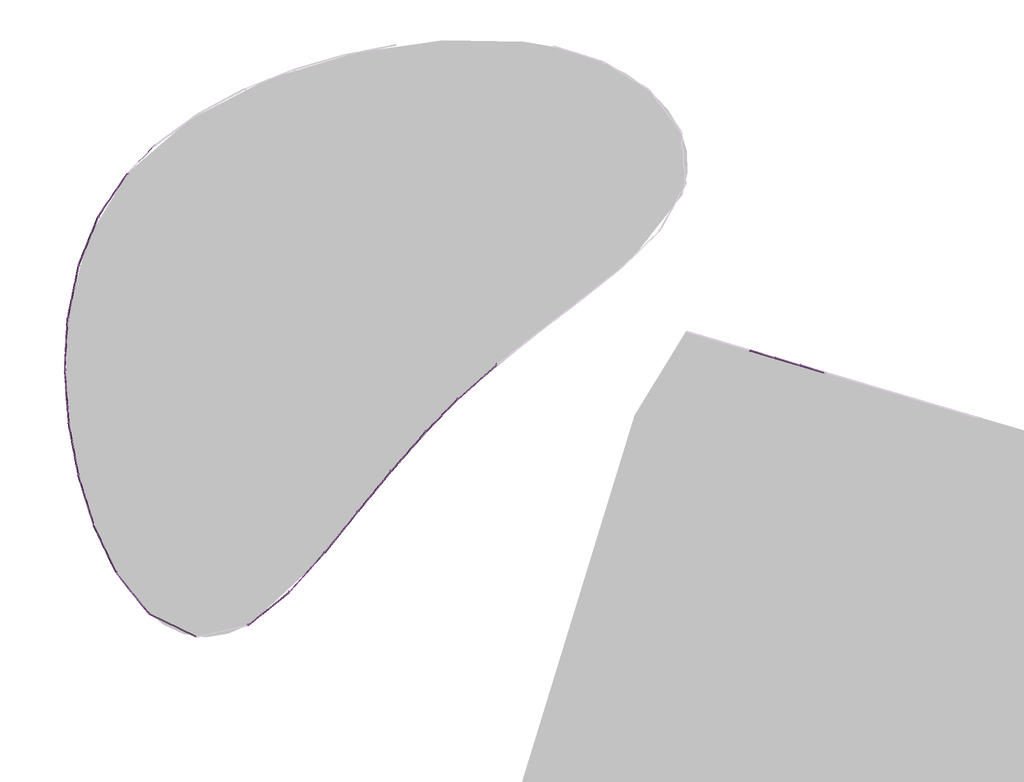
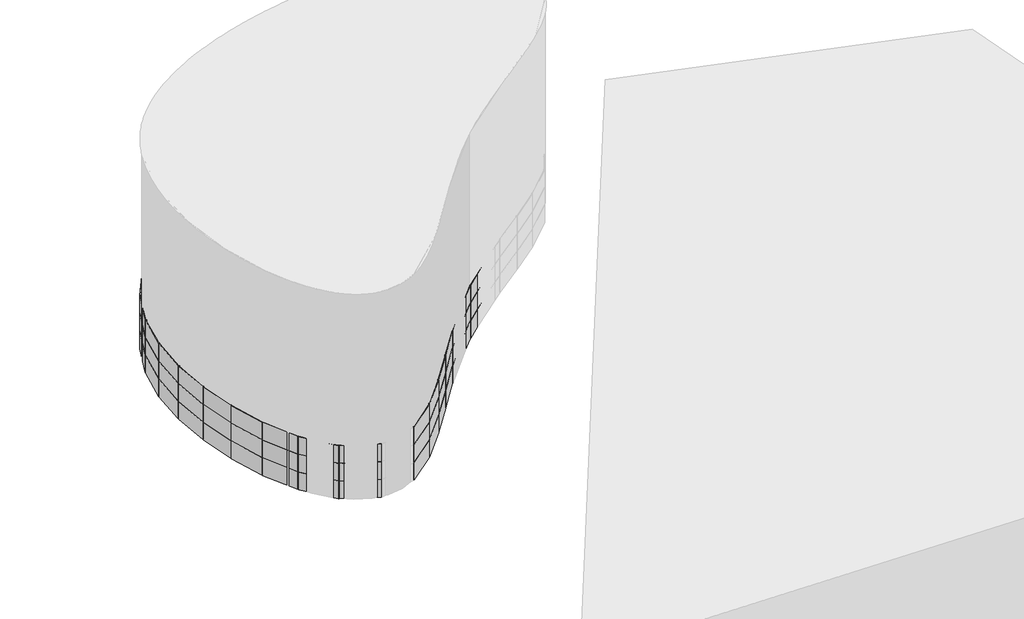
# One storey, part 3 of 5: 58 plates, 54 members.
"""IFC4 building model written with IfcOpenShell, lengths in millimetres."""

import ifcopenshell
import ifcopenshell.guid

model = None  # the IFC model being written
_history = None  # IfcOwnerHistory: only IFC2X3 demands one
_inside = {}  # id of a spatial element -> (the spatial element, [elements in it])
_under = {}  # id of a project, library or spatial element -> (it, [spatial elements below it])
_declared = {}  # id of a project -> (the project, [libraries it declares])
_typed = {}  # id of a type object -> (the type object, [elements of that type])
_made_of = {}  # id of a material, layer set ... -> (it, [elements and type objects made of it])


def new_model(schema):
    """Start an empty IFC model of exactly this schema.

    Asked for "IFC4X3", IfcOpenShell would pick the latest addendum, in which some entities
    have other attributes; the version numbers below select the first issue.
    IFC2X3 requires an IfcOwnerHistory on every rooted entity: one is made here for all.
    """
    global model, _history
    if schema == "IFC4X3":
        model = ifcopenshell.file(schema_version=(4, 3, 0, 0))
    else:
        model = ifcopenshell.file(schema=schema)
    _inside.clear()
    _under.clear()
    _declared.clear()
    _typed.clear()
    _made_of.clear()
    _history = None
    if model.schema == "IFC2X3":
        org = make("IfcOrganization", Name="unknown")
        user = make(
            "IfcPersonAndOrganization",
            ThePerson=make("IfcPerson", FamilyName="unknown"),
            TheOrganization=org,
        )
        app = make(
            "IfcApplication",
            ApplicationDeveloper=org,
            Version="unknown",
            ApplicationFullName="unknown",
            ApplicationIdentifier="unknown",
        )
        _history = make(
            "IfcOwnerHistory",
            OwningUser=user,
            OwningApplication=app,
            ChangeAction="ADDED",
            CreationDate=0,
        )
    return model


def make(cls, **values):
    """One entity of the class cls with the attributes given. An attribute that is None is left unset."""
    return model.create_entity(
        cls, **{name: value for name, value in values.items() if value is not None}
    )


def rooted(cls, **values):
    """An entity with a GlobalId (a new one), such as an element, a storey or a relation."""
    return make(cls, GlobalId=ifcopenshell.guid.new(), OwnerHistory=_history, **values)


def si_unit(unit_type, name, prefix=None):
    """IfcSIUnit, for example si_unit("LENGTHUNIT", "METRE", prefix="MILLI")."""
    return make("IfcSIUnit", UnitType=unit_type, Prefix=prefix, Name=name)


def assignment(units):
    """IfcUnitAssignment: the units of a project."""
    return None if units is None else make("IfcUnitAssignment", Units=units)


def point(xyz):
    """IfcCartesianPoint."""
    return None if xyz is None else make("IfcCartesianPoint", Coordinates=xyz)


def direction(xyz):
    """IfcDirection."""
    return None if xyz is None else make("IfcDirection", DirectionRatios=xyz)


def frame(location, z_axis=None, x_axis=None):
    """IfcAxis2Placement3D, a coordinate frame: its origin and axes. An axis left out is left unset."""
    return make(
        "IfcAxis2Placement3D",
        Location=point(location),
        Axis=direction(z_axis),
        RefDirection=direction(x_axis),
    )


def frame_2d(location, x_axis=None):
    """IfcAxis2Placement2D, a coordinate frame in the plane: its origin and x axis."""
    return make(
        "IfcAxis2Placement2D", Location=point(location), RefDirection=direction(x_axis)
    )


def origin():
    """The frame at (0, 0, 0) with its axes left unset."""
    return frame((0.0, 0.0, 0.0))


def origin_with_axes():
    """The frame at (0, 0, 0) with the z axis (0, 0, 1) and the x axis (1, 0, 0) written out."""
    return frame((0.0, 0.0, 0.0), z_axis=(0.0, 0.0, 1.0), x_axis=(1.0, 0.0, 0.0))


def origin_2d():
    """The frame at (0, 0) in the plane with its x axis left unset."""
    return frame_2d((0.0, 0.0))


def place(relative_to, where):
    """IfcLocalPlacement: puts the frame where relative to a parent placement (None: the world)."""
    return make(
        "IfcLocalPlacement", PlacementRelTo=relative_to, RelativePlacement=where
    )


def context(
    kind, dimensions, precision=None, world=None, true_north=None, identifier=None
):
    """IfcGeometricRepresentationContext, for example the 3D "Model" context."""
    return make(
        "IfcGeometricRepresentationContext",
        ContextIdentifier=identifier,
        ContextType=kind,
        CoordinateSpaceDimension=dimensions,
        Precision=precision,
        WorldCoordinateSystem=world,
        TrueNorth=true_north,
    )


def project(units=None, contexts=None):
    """IfcProject with its units and contexts."""
    return rooted(
        "IfcProject",
        Name="project",
        RepresentationContexts=contexts,
        UnitsInContext=assignment(units),
    )


def spatial(cls, under=None, at=None, **own):
    """A site, building, storey or space (cls), placed at a placement, below another one or the project."""
    s = rooted(cls, ObjectPlacement=at, **own)
    if under is not None:
        _under.setdefault(under.id(), (under, []))[1].append(s)
    return s


def polyline(points):
    """IfcPolyline through the points."""
    return make("IfcPolyline", Points=[point(p) for p in points])


def circle_curve(where, radius):
    """IfcCircle in the frame where."""
    return make("IfcCircle", Position=where, Radius=radius)


def trimmed(basis, trim1, trim2, sense, master):
    """IfcTrimmedCurve: the piece of a basis curve between two trims."""
    return make(
        "IfcTrimmedCurve",
        BasisCurve=basis,
        Trim1=trim1,
        Trim2=trim2,
        SenseAgreement=sense,
        MasterRepresentation=master,
    )


def segment(curve, same_sense, transition):
    """IfcCompositeCurveSegment."""
    return make(
        "IfcCompositeCurveSegment",
        Transition=transition,
        SameSense=same_sense,
        ParentCurve=curve,
    )


def composite_curve(segments, self_intersect=None):
    """IfcCompositeCurve: segments joined end to end."""
    return make("IfcCompositeCurve", Segments=segments, SelfIntersect=self_intersect)


def outline(outer, holes=None, kind="AREA"):
    """IfcArbitraryClosedProfileDef: a profile drawn as a closed curve; with holes, ...WithVoids."""
    if holes is None:
        return make("IfcArbitraryClosedProfileDef", ProfileType=kind, OuterCurve=outer)
    return make(
        "IfcArbitraryProfileDefWithVoids",
        ProfileType=kind,
        OuterCurve=outer,
        InnerCurves=holes,
    )


def extrude(swept, where, along, depth):
    """IfcExtrudedAreaSolid: the profile swept, set in the frame where, extruded along a direction by depth."""
    return make(
        "IfcExtrudedAreaSolid",
        SweptArea=swept,
        Position=where,
        ExtrudedDirection=direction(along),
        Depth=depth,
    )


def shape(context_of_items, identifier, shape_type, items):
    """IfcShapeRepresentation: the items that make up one representation, for example the "Body"."""
    return make(
        "IfcShapeRepresentation",
        ContextOfItems=context_of_items,
        RepresentationIdentifier=identifier,
        RepresentationType=shape_type,
        Items=items,
    )


def source(mapping_origin, context_of_items, identifier, shape_type, items):
    """IfcRepresentationMap: a shape defined once, which mapped items show again and again."""
    return make(
        "IfcRepresentationMap",
        MappingOrigin=mapping_origin,
        MappedRepresentation=shape(context_of_items, identifier, shape_type, items),
    )


def transform(
    local_origin,
    x_axis=None,
    y_axis=None,
    z_axis=None,
    scale=None,
    scale2=None,
    scale3=None,
    uniform=True,
):
    """IfcCartesianTransformationOperator3D, or its non-uniform kind. x_axis, y_axis, z_axis: its Axis1, 2, 3."""
    if uniform:
        return make(
            "IfcCartesianTransformationOperator3D",
            Axis1=direction(x_axis),
            Axis2=direction(y_axis),
            LocalOrigin=point(local_origin),
            Scale=scale,
            Axis3=direction(z_axis),
        )
    return make(
        "IfcCartesianTransformationOperator3DnonUniform",
        Axis1=direction(x_axis),
        Axis2=direction(y_axis),
        LocalOrigin=point(local_origin),
        Scale=scale,
        Axis3=direction(z_axis),
        Scale2=scale2,
        Scale3=scale3,
    )


def mapped(mapping_source, mapping_target):
    """IfcMappedItem: shows the shape of a source again, moved by a transform."""
    return make(
        "IfcMappedItem", MappingSource=mapping_source, MappingTarget=mapping_target
    )


def made_of(thing, what):
    """Note that an element or type object is made of a material, layer set ...; save() writes the relation."""
    if what is not None:
        _made_of.setdefault(what.id(), (what, []))[1].append(thing)
    return thing


def element(
    cls,
    number,
    at=None,
    inside=None,
    cuts=None,
    type_object=None,
    material=None,
    context=None,
    identifier="Body",
    shape_type=None,
    held_by="IfcProductDefinitionShape",
    body=None,
    shapes=None,
    **own,
):
    """One element of the class cls, such as IfcWall. Its Tag is "e" and its number.

    at: its placement. inside: the storey or other place that contains it. cuts: it is an
    opening in that element (IfcRelVoidsElement). A single representation is given by context,
    identifier, shape_type and body (its items); several are given by shapes. held_by: the class
    of the entity that holds the representations. save() writes the other relations.
    """
    e = rooted(cls, Tag="e%d" % number, ObjectPlacement=at, **own)
    if body is not None:
        shapes = [shape(context, identifier, shape_type, body)]
    if shapes is not None:
        e.Representation = make(held_by, Representations=shapes)
    if inside is not None:
        _inside.setdefault(inside.id(), (inside, []))[1].append(e)
    if cuts is not None:
        rooted(
            "IfcRelVoidsElement", RelatingBuildingElement=cuts, RelatedOpeningElement=e
        )
    if type_object is not None:
        _typed.setdefault(type_object.id(), (type_object, []))[1].append(e)
    return made_of(e, material)


def aggregate(whole, parts):
    """IfcRelAggregates: a whole, such as a stair, and the parts it consists of."""
    return rooted("IfcRelAggregates", RelatingObject=whole, RelatedObjects=parts)


def save(model, path):
    """Write the relations noted so far, then the file.

    IfcRelAggregates (storeys below a building ...), IfcRelContainedInSpatialStructure (elements
    in a storey), IfcRelDefinesByType, IfcRelAssociatesMaterial and IfcRelDeclares: one each for
    every whole, place, type object, material and project.
    """
    for whole, parts in _under.values():
        aggregate(whole, parts)
    for where, things in _inside.values():
        rooted(
            "IfcRelContainedInSpatialStructure",
            RelatedElements=things,
            RelatingStructure=where,
        )
    for kind, things in _typed.values():
        rooted("IfcRelDefinesByType", RelatedObjects=things, RelatingType=kind)
    for what, things in _made_of.values():
        rooted("IfcRelAssociatesMaterial", RelatedObjects=things, RelatingMaterial=what)
    for by, libraries in _declared.values():
        rooted("IfcRelDeclares", RelatingContext=by, RelatedDefinitions=libraries)
    model.write(path)


def montante_circular_25_mm_raio_36e581cf(model_context):
    return source(origin(), model_context, "Body", "SweptSolid", [
        extrude(outline(composite_curve([segment(trimmed(circle_curve(origin_2d(), 25.0), [point((25.0, 0.0))], [point((-25.0, 0.0))], False, "CARTESIAN"), True, "CONTINUOUS"), segment(trimmed(circle_curve(origin_2d(), 25.0), [point((-25.0, 0.0))], [point((25.0, 0.0))], False, "CARTESIAN"), True, "CONTINUOUS")], self_intersect=False)), frame((0.0, 0.0, -1500.0), z_axis=(0.0, 0.0, 1.0), x_axis=(1.0, 0.0, 0.0)), (0.0, 0.0, 1.0), 1500.0),
    ])


def montante_circular_25_mm_raio_ce826986(model_context):
    return source(origin(), model_context, "Body", "SweptSolid", [
        extrude(outline(composite_curve([segment(trimmed(circle_curve(frame_2d((-25.0, 0.0)), 25.0), [point((0.0, 0.0))], [point((-50.0, 0.0))], False, "CARTESIAN"), True, "CONTINUOUS"), segment(trimmed(circle_curve(frame_2d((-25.0, 0.0)), 25.0), [point((-50.0, 0.0))], [point((0.0, 0.0))], False, "CARTESIAN"), True, "CONTINUOUS")], self_intersect=False)), frame((0.0, 0.0, -1500.0), z_axis=(0.0, 0.0, 1.0), x_axis=(1.0, 0.0, 0.0)), (0.0, 0.0, 1.0), 1500.0),
    ])


def painel_do_sistema_ee4f1c4d(model_context):
    return source(origin(), model_context, "Body", "SweptSolid", [
        extrude(outline(polyline([(1487.5000075, 24.5), (-1487.5000075, 24.5), (-1487.5000075, 49.5), (1487.5000075, 49.5), (1487.5000075, 24.5)])), origin_with_axes(), (0.0, 0.0, 1.0), 1500.0),
    ])


def painel_do_sistema_5ef9eced(model_context):
    return source(origin(), model_context, "Body", "SweptSolid", [
        extrude(outline(polyline([(1475.0, 24.5), (-1475.0, 24.5), (-1475.0, 49.5), (1475.0, 49.5), (1475.0, 24.5)])), origin_with_axes(), (0.0, 0.0, 1.0), 1500.0),
    ])


def painel_do_sistema_619734db(model_context):
    return source(origin(), model_context, "Body", "SweptSolid", [
        extrude(outline(polyline([(1462.5000305, -49.5), (-1462.5000305, -49.5), (-1462.5000305, -24.5), (1462.5000305, -24.5), (1462.5000305, -49.5)])), origin_with_axes(), (0.0, 0.0, 1.0), 1500.0),
    ])


def painel_do_sistema_9c2734b9(model_context):
    return source(origin(), model_context, "Body", "SweptSolid", [
        extrude(outline(polyline([(1462.5000336, -49.5), (-1462.5000336, -49.5), (-1462.5000336, -24.5), (1462.5000336, -24.5), (1462.5000336, -49.5)])), origin_with_axes(), (0.0, 0.0, 1.0), 1500.0),
    ])


def painel_do_sistema_85ccde5d(model_context):
    return source(origin(), model_context, "Body", "SweptSolid", [
        extrude(outline(polyline([(1475.0, -49.5), (-1475.0, -49.5), (-1475.0, -24.5), (1475.0, -24.5), (1475.0, -49.5)])), origin_with_axes(), (0.0, 0.0, 1.0), 1500.0),
    ])


def painel_do_sistema_91df381f(model_context):
    return source(origin(), model_context, "Body", "SweptSolid", [
        extrude(outline(polyline([(1110.3819696, -49.5), (-1110.3819696, -49.5), (-1110.3819696, -24.5), (1110.3819696, -24.5), (1110.3819696, -49.5)])), origin_with_axes(), (0.0, 0.0, 1.0), 1500.0),
    ])


def painel_do_sistema_bfc8fefc(model_context):
    return source(origin(), model_context, "Body", "SweptSolid", [
        extrude(outline(polyline([(1275.8375317, -49.5), (-1275.8375317, -49.5), (-1275.8375317, -24.5), (1275.8375317, -24.5), (1275.8375317, -49.5)])), origin_with_axes(), (0.0, 0.0, 1.0), 1500.0),
    ])


model = new_model("IFC4")

# Units and contexts
model_context = context("Model", 3, world=origin())
ifc_project = project(units=[si_unit("LENGTHUNIT", "METRE", prefix="MILLI")], contexts=[model_context])

# Site, building, storey
site = spatial("IfcSite", under=ifc_project)
building = spatial("IfcBuilding", under=site)
storey = spatial("IfcBuildingStorey", under=building, Name="Nível 1", Elevation=0.0)

# Members
placement = place(None, origin())
montante_circular_25_mm_raio_shape = montante_circular_25_mm_raio_36e581cf(model_context)
element("IfcMember", 1, ObjectType="Montante circular : 25 mm Raio", at=placement, inside=storey, context=model_context, shape_type="MappedRepresentation", body=[
    mapped(montante_circular_25_mm_raio_shape, transform((-73.9726554, 31091.8210426, 3000.000015), x_axis=(0.0, 0.0, 1.0), y_axis=(0.28318378939534855, 0.9590656606425293, 0.0), z_axis=(-0.9590656606425293, 0.28318378939534855, 0.0))),
])
element("IfcMember", 2, ObjectType="Montante circular : 25 mm Raio", at=placement, inside=storey, context=model_context, shape_type="MappedRepresentation", body=[
    mapped(montante_circular_25_mm_raio_shape, transform((-1512.5711463, 31516.5967267, 3000.000015), x_axis=(0.0, 0.0, 1.0), y_axis=(0.28318378939534655, 0.9590656606425297, 0.0), z_axis=(-0.9590656606425296, 0.2831837893953465, 0.0))),
])
element("IfcMember", 3, ObjectType="Montante circular : 25 mm Raio", at=placement, inside=storey, context=model_context, shape_type="MappedRepresentation", body=[
    mapped(montante_circular_25_mm_raio_shape, transform((-2951.1696373, 31941.3724108, 3000.000015), x_axis=(0.0, 0.0, 1.0), y_axis=(0.2831837893953519, 0.9590656606425282, 0.0), z_axis=(-0.9590656606425281, 0.2831837893953518, 0.0))),
])
element("IfcMember", 4, ObjectType="Montante circular : 25 mm Raio", at=placement, inside=storey, context=model_context, shape_type="MappedRepresentation", body=[
    mapped(montante_circular_25_mm_raio_shape, transform((-40020.7762885, 39520.8946952, 1500.0), x_axis=(-0.46558849269393926, -0.8850013307735677, 0.0), y_axis=(-0.8850013307735677, 0.46558849269393926, 0.0), z_axis=(0.0, 0.0, -1.0))),
])
element("IfcMember", 5, ObjectType="Montante circular : 25 mm Raio", at=placement, inside=storey, context=model_context, shape_type="MappedRepresentation", body=[
    mapped(montante_circular_25_mm_raio_shape, transform((-41145.2595981, 36739.6113068, 1500.0), x_axis=(-0.2854090553713671, -0.9584057966811469, 0.0), y_axis=(-0.9584057966811469, 0.2854090553713671, 0.0), z_axis=(0.0, 0.0, -1.0))),
])
element("IfcMember", 6, ObjectType="Montante circular : 25 mm Raio", at=placement, inside=storey, context=model_context, shape_type="MappedRepresentation", body=[
    mapped(montante_circular_25_mm_raio_shape, transform((-41757.3897475, 33802.725766, 1500.0), x_axis=(-0.12631233821712984, -0.9919905207279561, 0.0), y_axis=(-0.9919905207279561, 0.12631233821712984, 0.0), z_axis=(0.0, 0.0, -1.0))),
])
element("IfcMember", 7, ObjectType="Montante circular : 25 mm Raio", at=placement, inside=storey, context=model_context, shape_type="MappedRepresentation", body=[
    mapped(montante_circular_25_mm_raio_shape, transform((-41927.7364355, 30807.566003, 1500.0), x_axis=(0.00926833746122375, -0.999957048037917, 0.0), y_axis=(-0.999957048037917, -0.00926833746122375, 0.0), z_axis=(0.0, 0.0, -1.0))),
])
element("IfcMember", 8, ObjectType="Montante circular : 25 mm Raio", at=placement, inside=storey, context=model_context, shape_type="MappedRepresentation", body=[
    mapped(montante_circular_25_mm_raio_shape, transform((-41719.5366875, 27814.7992454, 1500.0), x_axis=(0.12720739477424994, -0.9918761408133316, 0.0), y_axis=(-0.9918761408133316, -0.12720739477424994, 0.0), z_axis=(0.0, 0.0, -1.0))),
])
element("IfcMember", 9, ObjectType="Montante circular : 25 mm Raio", at=placement, inside=storey, context=model_context, shape_type="MappedRepresentation", body=[
    mapped(montante_circular_25_mm_raio_shape, transform((-41172.4912602, 24865.0973452, 1500.0), x_axis=(0.2368789337610514, -0.9715391761222125, 0.0), y_axis=(-0.9715391761222125, -0.2368789337610514, 0.0), z_axis=(0.0, 0.0, -1.0))),
])
element("IfcMember", 10, ObjectType="Montante circular : 25 mm Raio", at=placement, inside=storey, context=model_context, shape_type="MappedRepresentation", body=[
    mapped(montante_circular_25_mm_raio_shape, transform((-39014.8508906, 19282.6093761, 1500.0), x_axis=(0.5079873162147127, -0.8613645491689181, 0.0), y_axis=(-0.8613645491689181, -0.5079873162147127, 0.0), z_axis=(0.0, 0.0, -1.0))),
])
element("IfcMember", 11, ObjectType="Montante circular : 25 mm Raio", at=placement, inside=storey, context=model_context, shape_type="MappedRepresentation", body=[
    mapped(montante_circular_25_mm_raio_shape, transform((-37150.2365801, 16932.4575783, 1500.0), x_axis=(0.7466685294931724, -0.665196292130754, 0.0), y_axis=(-0.665196292130754, -0.7466685294931724, 0.0), z_axis=(0.0, 0.0, -1.0))),
])
element("IfcMember", 12, ObjectType="Montante circular : 25 mm Raio", at=placement, inside=storey, context=model_context, shape_type="MappedRepresentation", body=[
    mapped(montante_circular_25_mm_raio_shape, transform((-31525.1733328, 16282.9834173, 1500.0), x_axis=(0.8701634838175947, 0.492763139277307, 0.0), y_axis=(0.492763139277307, -0.8701634838175947, 0.0), z_axis=(0.0, 0.0, -1.0))),
])
element("IfcMember", 13, ObjectType="Montante circular : 25 mm Raio", at=placement, inside=storey, context=model_context, shape_type="MappedRepresentation", body=[
    mapped(montante_circular_25_mm_raio_shape, transform((-29189.3459235, 18165.5110569, 1500.0), x_axis=(0.7046961293095542, 0.7095092426009207, 0.0), y_axis=(0.7095092426009207, -0.7046961293095542, 0.0), z_axis=(0.0, 0.0, -1.0))),
])
element("IfcMember", 14, ObjectType="Montante circular : 25 mm Raio", at=placement, inside=storey, context=model_context, shape_type="MappedRepresentation", body=[
    mapped(montante_circular_25_mm_raio_shape, transform((-27187.2576877, 20399.7095029, 1500.0), x_axis=(0.6410206876840714, 0.7675236009146822, 0.0), y_axis=(0.7675236009146822, -0.6410206876840714, 0.0), z_axis=(0.0, 0.0, -1.0))),
])
element("IfcMember", 15, ObjectType="Montante circular : 25 mm Raio", at=placement, inside=storey, context=model_context, shape_type="MappedRepresentation", body=[
    mapped(montante_circular_25_mm_raio_shape, transform((-25293.7553869, 22726.6493467, 1500.0), x_axis=(0.6272671926241681, 0.7788041275297628, 0.0), y_axis=(0.7788041275297628, -0.6272671926241681, 0.0), z_axis=(0.0, 0.0, -1.0))),
])
element("IfcMember", 16, ObjectType="Montante circular : 25 mm Raio", at=placement, inside=storey, context=model_context, shape_type="MappedRepresentation", body=[
    mapped(montante_circular_25_mm_raio_shape, transform((-23394.8086307, 25049.1482632, 1500.0), x_axis=(0.6426798456549805, 0.7661348549628131, 0.0), y_axis=(0.7661348549628131, -0.6426798456549805, 0.0), z_axis=(0.0, 0.0, -1.0))),
])
element("IfcMember", 17, ObjectType="Montante circular : 25 mm Raio", at=placement, inside=storey, context=model_context, shape_type="MappedRepresentation", body=[
    mapped(montante_circular_25_mm_raio_shape, transform((-21416.0981725, 27304.0772915, 1500.0), x_axis=(0.6795654424505699, 0.7336148917701719, 0.0), y_axis=(0.7336148917701719, -0.6795654424505699, 0.0), z_axis=(0.0, 0.0, -1.0))),
])
element("IfcMember", 18, ObjectType="Montante circular : 25 mm Raio", at=placement, inside=storey, context=model_context, shape_type="MappedRepresentation", body=[
    mapped(montante_circular_25_mm_raio_shape, transform((-40020.7762885, 39520.8946952, 3000.0), x_axis=(-0.46558849269393926, -0.8850013307735677, 0.0), y_axis=(-0.8850013307735677, 0.46558849269393926, 0.0), z_axis=(0.0, 0.0, -1.0))),
])
element("IfcMember", 19, ObjectType="Montante circular : 25 mm Raio", at=placement, inside=storey, context=model_context, shape_type="MappedRepresentation", body=[
    mapped(montante_circular_25_mm_raio_shape, transform((-41145.2595981, 36739.6113068, 3000.0), x_axis=(-0.28540905537136685, -0.958405796681147, 0.0), y_axis=(-0.958405796681147, 0.28540905537136685, 0.0), z_axis=(0.0, 0.0, -1.0))),
])
element("IfcMember", 20, ObjectType="Montante circular : 25 mm Raio", at=placement, inside=storey, context=model_context, shape_type="MappedRepresentation", body=[
    mapped(montante_circular_25_mm_raio_shape, transform((-41757.3897475, 33802.725766, 3000.0), x_axis=(-0.12631233821712995, -0.9919905207279561, 0.0), y_axis=(-0.9919905207279561, 0.12631233821712995, 0.0), z_axis=(0.0, 0.0, -1.0))),
])
element("IfcMember", 21, ObjectType="Montante circular : 25 mm Raio", at=placement, inside=storey, context=model_context, shape_type="MappedRepresentation", body=[
    mapped(montante_circular_25_mm_raio_shape, transform((-41927.7364355, 30807.566003, 3000.0), x_axis=(0.009268337461223748, -0.999957048037917, 0.0), y_axis=(-0.999957048037917, -0.009268337461223748, 0.0), z_axis=(0.0, 0.0, -1.0))),
])
element("IfcMember", 22, ObjectType="Montante circular : 25 mm Raio", at=placement, inside=storey, context=model_context, shape_type="MappedRepresentation", body=[
    mapped(montante_circular_25_mm_raio_shape, transform((-41719.5366875, 27814.7992454, 3000.0), x_axis=(0.12720739477424994, -0.9918761408133316, 0.0), y_axis=(-0.9918761408133316, -0.12720739477424994, 0.0), z_axis=(0.0, 0.0, -1.0))),
])
element("IfcMember", 23, ObjectType="Montante circular : 25 mm Raio", at=placement, inside=storey, context=model_context, shape_type="MappedRepresentation", body=[
    mapped(montante_circular_25_mm_raio_shape, transform((-41172.4912602, 24865.0973452, 3000.0), x_axis=(0.23687893376105149, -0.9715391761222125, 0.0), y_axis=(-0.9715391761222125, -0.23687893376105149, 0.0), z_axis=(0.0, 0.0, -1.0))),
])
element("IfcMember", 24, ObjectType="Montante circular : 25 mm Raio", at=placement, inside=storey, context=model_context, shape_type="MappedRepresentation", body=[
    mapped(montante_circular_25_mm_raio_shape, transform((-39014.8508906, 19282.6093761, 3000.0), x_axis=(0.5079873162147126, -0.8613645491689182, 0.0), y_axis=(-0.8613645491689182, -0.5079873162147126, 0.0), z_axis=(0.0, 0.0, -1.0))),
])
element("IfcMember", 25, ObjectType="Montante circular : 25 mm Raio", at=placement, inside=storey, context=model_context, shape_type="MappedRepresentation", body=[
    mapped(montante_circular_25_mm_raio_shape, transform((-37150.2365801, 16932.4575783, 3000.0), x_axis=(0.7466685294931728, -0.6651962921307538, 0.0), y_axis=(-0.6651962921307538, -0.7466685294931728, 0.0), z_axis=(0.0, 0.0, -1.0))),
])
element("IfcMember", 26, ObjectType="Montante circular : 25 mm Raio", at=placement, inside=storey, context=model_context, shape_type="MappedRepresentation", body=[
    mapped(montante_circular_25_mm_raio_shape, transform((-31525.1733328, 16282.9834173, 3000.0), x_axis=(0.8701634838175948, 0.49276313927730697, 0.0), y_axis=(0.49276313927730697, -0.8701634838175948, 0.0), z_axis=(0.0, 0.0, -1.0))),
])
element("IfcMember", 27, ObjectType="Montante circular : 25 mm Raio", at=placement, inside=storey, context=model_context, shape_type="MappedRepresentation", body=[
    mapped(montante_circular_25_mm_raio_shape, transform((-29189.3459235, 18165.5110569, 3000.0), x_axis=(0.7046961293095542, 0.7095092426009207, 0.0), y_axis=(0.7095092426009207, -0.7046961293095542, 0.0), z_axis=(0.0, 0.0, -1.0))),
])
element("IfcMember", 28, ObjectType="Montante circular : 25 mm Raio", at=placement, inside=storey, context=model_context, shape_type="MappedRepresentation", body=[
    mapped(montante_circular_25_mm_raio_shape, transform((-27187.2576877, 20399.7095029, 3000.0), x_axis=(0.6410206876840713, 0.7675236009146822, 0.0), y_axis=(0.7675236009146822, -0.6410206876840713, 0.0), z_axis=(0.0, 0.0, -1.0))),
])
element("IfcMember", 29, ObjectType="Montante circular : 25 mm Raio", at=placement, inside=storey, context=model_context, shape_type="MappedRepresentation", body=[
    mapped(montante_circular_25_mm_raio_shape, transform((-25293.7553869, 22726.6493467, 3000.0), x_axis=(0.627267192624168, 0.7788041275297628, 0.0), y_axis=(0.7788041275297628, -0.627267192624168, 0.0), z_axis=(0.0, 0.0, -1.0))),
])
element("IfcMember", 30, ObjectType="Montante circular : 25 mm Raio", at=placement, inside=storey, context=model_context, shape_type="MappedRepresentation", body=[
    mapped(montante_circular_25_mm_raio_shape, transform((-23394.8086307, 25049.1482632, 3000.0), x_axis=(0.6426798456549805, 0.766134854962813, 0.0), y_axis=(0.766134854962813, -0.6426798456549805, 0.0), z_axis=(0.0, 0.0, -1.0))),
])
element("IfcMember", 31, ObjectType="Montante circular : 25 mm Raio", at=placement, inside=storey, context=model_context, shape_type="MappedRepresentation", body=[
    mapped(montante_circular_25_mm_raio_shape, transform((-21416.0981725, 27304.0772915, 3000.0), x_axis=(0.67956544245057, 0.7336148917701719, 0.0), y_axis=(0.7336148917701719, -0.67956544245057, 0.0), z_axis=(0.0, 0.0, -1.0))),
])
element("IfcMember", 32, ObjectType="Montante circular : 25 mm Raio", at=placement, inside=storey, context=model_context, shape_type="MappedRepresentation", body=[
    mapped(montante_circular_25_mm_raio_shape, transform((-17353.3233761, 31118.8559936, 1500.0), x_axis=(0.7724767966577649, 0.6350429895883886, 0.0), y_axis=(0.6350429895883886, -0.7724767966577649, 0.0), z_axis=(0.0, 0.0, -1.0))),
])
element("IfcMember", 33, ObjectType="Montante circular : 25 mm Raio", at=placement, inside=storey, context=model_context, shape_type="MappedRepresentation", body=[
    mapped(montante_circular_25_mm_raio_shape, transform((-17353.3233761, 31118.8559936, 3000.0), x_axis=(0.7724767966577649, 0.6350429895883886, 0.0), y_axis=(0.6350429895883886, -0.7724767966577649, 0.0), z_axis=(0.0, 0.0, -1.0))),
])
element("IfcMember", 34, ObjectType="Montante circular : 25 mm Raio", at=placement, inside=storey, context=model_context, shape_type="MappedRepresentation", body=[
    mapped(montante_circular_25_mm_raio_shape, transform((-40020.7762885, 39520.8946952, 0.0), x_axis=(-0.4655884926939391, -0.8850013307735677, 0.0), y_axis=(-0.8850013307735677, 0.4655884926939391, 0.0), z_axis=(0.0, 0.0, -1.0))),
])
element("IfcMember", 35, ObjectType="Montante circular : 25 mm Raio", at=placement, inside=storey, context=model_context, shape_type="MappedRepresentation", body=[
    mapped(montante_circular_25_mm_raio_shape, transform((-41145.2595981, 36739.6113068, 0.0), x_axis=(-0.28540905537136674, -0.958405796681147, 0.0), y_axis=(-0.958405796681147, 0.28540905537136674, 0.0), z_axis=(0.0, 0.0, -1.0))),
])
element("IfcMember", 36, ObjectType="Montante circular : 25 mm Raio", at=placement, inside=storey, context=model_context, shape_type="MappedRepresentation", body=[
    mapped(montante_circular_25_mm_raio_shape, transform((-41757.3897475, 33802.725766, 0.0), x_axis=(-0.12631233821712995, -0.9919905207279561, 0.0), y_axis=(-0.9919905207279561, 0.12631233821712995, 0.0), z_axis=(0.0, 0.0, -1.0))),
])
element("IfcMember", 37, ObjectType="Montante circular : 25 mm Raio", at=placement, inside=storey, context=model_context, shape_type="MappedRepresentation", body=[
    mapped(montante_circular_25_mm_raio_shape, transform((-41927.7364355, 30807.566003, 0.0), x_axis=(0.00926833746122375, -0.999957048037917, 0.0), y_axis=(-0.999957048037917, -0.00926833746122375, 0.0), z_axis=(0.0, 0.0, -1.0))),
])
element("IfcMember", 38, ObjectType="Montante circular : 25 mm Raio", at=placement, inside=storey, context=model_context, shape_type="MappedRepresentation", body=[
    mapped(montante_circular_25_mm_raio_shape, transform((-41719.5366875, 27814.7992454, 0.0), x_axis=(0.12720739477424994, -0.9918761408133316, 0.0), y_axis=(-0.9918761408133316, -0.12720739477424994, 0.0), z_axis=(0.0, 0.0, -1.0))),
])
element("IfcMember", 39, ObjectType="Montante circular : 25 mm Raio", at=placement, inside=storey, context=model_context, shape_type="MappedRepresentation", body=[
    mapped(montante_circular_25_mm_raio_shape, transform((-41172.4912602, 24865.0973452, 0.0), x_axis=(0.23687893376105146, -0.9715391761222125, 0.0), y_axis=(-0.9715391761222125, -0.23687893376105146, 0.0), z_axis=(0.0, 0.0, -1.0))),
])
element("IfcMember", 40, ObjectType="Montante circular : 25 mm Raio", at=placement, inside=storey, context=model_context, shape_type="MappedRepresentation", body=[
    mapped(montante_circular_25_mm_raio_shape, transform((-39014.8508906, 19282.6093761, 0.0), x_axis=(0.5079873162147126, -0.8613645491689182, 0.0), y_axis=(-0.8613645491689182, -0.5079873162147126, 0.0), z_axis=(0.0, 0.0, -1.0))),
])
element("IfcMember", 41, ObjectType="Montante circular : 25 mm Raio", at=placement, inside=storey, context=model_context, shape_type="MappedRepresentation", body=[
    mapped(montante_circular_25_mm_raio_shape, transform((-37150.2365801, 16932.4575783, 0.0), x_axis=(0.7466685294931728, -0.6651962921307538, 0.0), y_axis=(-0.6651962921307538, -0.7466685294931728, 0.0), z_axis=(0.0, 0.0, -1.0))),
])
element("IfcMember", 42, ObjectType="Montante circular : 25 mm Raio", at=placement, inside=storey, context=model_context, shape_type="MappedRepresentation", body=[
    mapped(montante_circular_25_mm_raio_shape, transform((-31525.1733328, 16282.9834173, 0.0), x_axis=(0.870163483817595, 0.49276313927730647, 0.0), y_axis=(0.49276313927730647, -0.870163483817595, 0.0), z_axis=(0.0, 0.0, -1.0))),
])
element("IfcMember", 43, ObjectType="Montante circular : 25 mm Raio", at=placement, inside=storey, context=model_context, shape_type="MappedRepresentation", body=[
    mapped(montante_circular_25_mm_raio_shape, transform((-29189.3459235, 18165.5110569, 0.0), x_axis=(0.7046961293095542, 0.7095092426009207, 0.0), y_axis=(0.7095092426009207, -0.7046961293095542, 0.0), z_axis=(0.0, 0.0, -1.0))),
])
element("IfcMember", 44, ObjectType="Montante circular : 25 mm Raio", at=placement, inside=storey, context=model_context, shape_type="MappedRepresentation", body=[
    mapped(montante_circular_25_mm_raio_shape, transform((-27187.2576877, 20399.7095029, 0.0), x_axis=(0.6410206876840713, 0.7675236009146822, 0.0), y_axis=(0.7675236009146822, -0.6410206876840713, 0.0), z_axis=(0.0, 0.0, -1.0))),
])
element("IfcMember", 45, ObjectType="Montante circular : 25 mm Raio", at=placement, inside=storey, context=model_context, shape_type="MappedRepresentation", body=[
    mapped(montante_circular_25_mm_raio_shape, transform((-25293.7553869, 22726.6493467, 0.0), x_axis=(0.627267192624168, 0.7788041275297628, 0.0), y_axis=(0.7788041275297628, -0.627267192624168, 0.0), z_axis=(0.0, 0.0, -1.0))),
])
element("IfcMember", 46, ObjectType="Montante circular : 25 mm Raio", at=placement, inside=storey, context=model_context, shape_type="MappedRepresentation", body=[
    mapped(montante_circular_25_mm_raio_shape, transform((-23394.8086307, 25049.1482632, 0.0), x_axis=(0.6426798456549805, 0.766134854962813, 0.0), y_axis=(0.766134854962813, -0.6426798456549805, 0.0), z_axis=(0.0, 0.0, -1.0))),
])
element("IfcMember", 47, ObjectType="Montante circular : 25 mm Raio", at=placement, inside=storey, context=model_context, shape_type="MappedRepresentation", body=[
    mapped(montante_circular_25_mm_raio_shape, transform((-21416.0981725, 27304.0772915, 0.0), x_axis=(0.6795654424505699, 0.7336148917701719, 0.0), y_axis=(0.7336148917701719, -0.6795654424505699, 0.0), z_axis=(0.0, 0.0, -1.0))),
])
element("IfcMember", 48, ObjectType="Montante circular : 25 mm Raio", at=placement, inside=storey, context=model_context, shape_type="MappedRepresentation", body=[
    mapped(montante_circular_25_mm_raio_shape, transform((-17353.3233761, 31118.8559936, 0.0), x_axis=(0.7724767966577648, 0.6350429895883886, 0.0), y_axis=(0.6350429895883886, -0.7724767966577648, 0.0), z_axis=(0.0, 0.0, -1.0))),
])
montante_circular_25_mm_raio_2_shape = montante_circular_25_mm_raio_ce826986(model_context)
element("IfcMember", 49, ObjectType="Montante circular : 25 mm Raio", at=placement, inside=storey, context=model_context, shape_type="MappedRepresentation", body=[
    mapped(montante_circular_25_mm_raio_2_shape, transform((-38343.4953128, 42008.2082927, 1500.0), x_axis=(0.5590936460250591, 0.829104513903046, 0.0), y_axis=(-0.829104513903046, 0.5590936460250591, 0.0), z_axis=(0.0, 0.0, 1.0))),
])
element("IfcMember", 50, ObjectType="Montante circular : 25 mm Raio", at=placement, inside=storey, context=model_context, shape_type="MappedRepresentation", body=[
    mapped(montante_circular_25_mm_raio_2_shape, transform((-19607.9031675, 29139.747525, 1500.0), x_axis=(-0.7515265818306628, -0.659702809454318, 0.0), y_axis=(0.659702809454318, -0.7515265818306628, 0.0), z_axis=(0.0, 0.0, 1.0))),
])
element("IfcMember", 51, ObjectType="Montante circular : 25 mm Raio", at=placement, inside=storey, context=model_context, shape_type="MappedRepresentation", body=[
    mapped(montante_circular_25_mm_raio_2_shape, transform((-38343.4953128, 42008.2082927, 3000.0), x_axis=(0.5590936460250591, 0.829104513903046, 0.0), y_axis=(-0.829104513903046, 0.5590936460250591, 0.0), z_axis=(0.0, 0.0, 1.0))),
])
element("IfcMember", 52, ObjectType="Montante circular : 25 mm Raio", at=placement, inside=storey, context=model_context, shape_type="MappedRepresentation", body=[
    mapped(montante_circular_25_mm_raio_2_shape, transform((-38343.4953128, 42008.2082927, 4500.0), x_axis=(0.5590936460250591, 0.829104513903046, 0.0), y_axis=(-0.829104513903046, 0.5590936460250591, 0.0), z_axis=(0.0, 0.0, 1.0))),
])
element("IfcMember", 53, ObjectType="Montante circular : 25 mm Raio", at=placement, inside=storey, context=model_context, shape_type="MappedRepresentation", body=[
    mapped(montante_circular_25_mm_raio_2_shape, transform((-19607.9031675, 29139.747525, 3000.0), x_axis=(-0.7515265818306612, -0.6597028094543197, 0.0), y_axis=(0.6597028094543197, -0.7515265818306612, 0.0), z_axis=(0.0, 0.0, 1.0))),
])
element("IfcMember", 54, ObjectType="Montante circular : 25 mm Raio", at=placement, inside=storey, context=model_context, shape_type="MappedRepresentation", body=[
    mapped(montante_circular_25_mm_raio_2_shape, transform((-19607.9031675, 29139.747525, 4500.0), x_axis=(-0.7515265818306621, -0.6597028094543188, 0.0), y_axis=(0.6597028094543188, -0.7515265818306621, 0.0), z_axis=(0.0, 0.0, 1.0))),
])

# Plates
painel_do_sistema_shape = painel_do_sistema_ee4f1c4d(model_context)
element("IfcPlate", 55, ObjectType="Painel do sistema : Envidraçado", at=placement, inside=storey, context=model_context, shape_type="MappedRepresentation", body=[
    mapped(painel_do_sistema_shape, transform((-73.9726554, 31091.8210426, 1487.5000075), x_axis=(0.0, 0.0, 1.0), y_axis=(-0.2831837893953486, -0.9590656606425292, 0.0), z_axis=(0.9590656606425292, -0.2831837893953486, 0.0))),
])
element("IfcPlate", 56, ObjectType="Painel do sistema : Envidraçado", at=placement, inside=storey, context=model_context, shape_type="MappedRepresentation", body=[
    mapped(painel_do_sistema_shape, transform((-1512.5711463, 31516.5967267, 1487.5000075), x_axis=(0.0, 0.0, 1.0), y_axis=(-0.28318378939534655, -0.9590656606425297, 0.0), z_axis=(0.9590656606425297, -0.28318378939534655, 0.0))),
])
element("IfcPlate", 57, ObjectType="Painel do sistema : Envidraçado", at=placement, inside=storey, context=model_context, shape_type="MappedRepresentation", body=[
    mapped(painel_do_sistema_shape, transform((-2951.1696373, 31941.3724108, 1487.5000075), x_axis=(0.0, 0.0, 1.0), y_axis=(-0.2831837893953519, -0.9590656606425282, 0.0), z_axis=(0.9590656606425282, -0.2831837893953519, 0.0))),
])
painel_do_sistema_2_shape = painel_do_sistema_5ef9eced(model_context)
element("IfcPlate", 58, ObjectType="Painel do sistema : Envidraçado", at=placement, inside=storey, context=model_context, shape_type="MappedRepresentation", body=[
    mapped(painel_do_sistema_2_shape, transform((-73.9726554, 31091.8210426, 4500.00001), x_axis=(0.0, 0.0, 1.0), y_axis=(-0.2831837893953487, -0.9590656606425292, 0.0), z_axis=(0.9590656606425292, -0.2831837893953487, 0.0))),
])
element("IfcPlate", 59, ObjectType="Painel do sistema : Envidraçado", at=placement, inside=storey, context=model_context, shape_type="MappedRepresentation", body=[
    mapped(painel_do_sistema_2_shape, transform((-1512.5711463, 31516.5967267, 4500.00001), x_axis=(0.0, 0.0, 1.0), y_axis=(-0.2831837893953465, -0.9590656606425297, 0.0), z_axis=(0.9590656606425297, -0.2831837893953465, 0.0))),
])
element("IfcPlate", 60, ObjectType="Painel do sistema : Envidraçado", at=placement, inside=storey, context=model_context, shape_type="MappedRepresentation", body=[
    mapped(painel_do_sistema_2_shape, transform((-2951.1696373, 31941.3724108, 4500.00001), x_axis=(0.0, 0.0, 1.0), y_axis=(-0.2831837893953518, -0.9590656606425282, 0.0), z_axis=(0.9590656606425282, -0.2831837893953518, 0.0))),
])
painel_do_sistema_3_shape = painel_do_sistema_619734db(model_context)
element("IfcPlate", 61, ObjectType="Painel do sistema : Envidraçado", at=placement, inside=storey, context=model_context, shape_type="MappedRepresentation", body=[
    mapped(painel_do_sistema_3_shape, transform((-18471.2191895, 30137.5480444, 0.0), x_axis=(0.7515265818306628, 0.659702809454318, 0.0), y_axis=(-0.659702809454318, 0.7515265818306628, 0.0), z_axis=(0.0, 0.0, 1.0))),
])
element("IfcPlate", 62, ObjectType="Painel do sistema : Envidraçado", at=placement, inside=storey, context=model_context, shape_type="MappedRepresentation", body=[
    mapped(painel_do_sistema_3_shape, transform((-18471.2191895, 30137.5480444, 1500.0), x_axis=(0.7515265818306612, 0.6597028094543197, 0.0), y_axis=(-0.6597028094543197, 0.7515265818306612, 0.0), z_axis=(0.0, 0.0, 1.0))),
])
element("IfcPlate", 63, ObjectType="Painel do sistema : Envidraçado", at=placement, inside=storey, context=model_context, shape_type="MappedRepresentation", body=[
    mapped(painel_do_sistema_3_shape, transform((-18471.2191895, 30137.5480444, 3000.0), x_axis=(0.7515265818306621, 0.6597028094543188, 0.0), y_axis=(-0.6597028094543188, 0.7515265818306621, 0.0), z_axis=(0.0, 0.0, 1.0))),
])
painel_do_sistema_4_shape = painel_do_sistema_9c2734b9(model_context)
element("IfcPlate", 64, ObjectType="Painel do sistema : Envidraçado", at=placement, inside=storey, context=model_context, shape_type="MappedRepresentation", body=[
    mapped(painel_do_sistema_4_shape, transform((-39189.1244712, 40754.1876875, 0.0), x_axis=(-0.5590936460250591, -0.829104513903046, 0.0), y_axis=(0.829104513903046, -0.5590936460250591, 0.0), z_axis=(0.0, 0.0, 1.0))),
])
element("IfcPlate", 65, ObjectType="Painel do sistema : Envidraçado", at=placement, inside=storey, context=model_context, shape_type="MappedRepresentation", body=[
    mapped(painel_do_sistema_4_shape, transform((-39189.1244712, 40754.1876875, 1500.0), x_axis=(-0.5590936460250591, -0.829104513903046, 0.0), y_axis=(0.829104513903046, -0.5590936460250591, 0.0), z_axis=(0.0, 0.0, 1.0))),
])
element("IfcPlate", 66, ObjectType="Painel do sistema : Envidraçado", at=placement, inside=storey, context=model_context, shape_type="MappedRepresentation", body=[
    mapped(painel_do_sistema_4_shape, transform((-39189.1244712, 40754.1876875, 3000.0), x_axis=(-0.5590936460250591, -0.829104513903046, 0.0), y_axis=(0.829104513903046, -0.5590936460250591, 0.0), z_axis=(0.0, 0.0, 1.0))),
])
painel_do_sistema_5_shape = painel_do_sistema_85ccde5d(model_context)
element("IfcPlate", 67, ObjectType="Painel do sistema : Envidraçado", at=placement, inside=storey, context=model_context, shape_type="MappedRepresentation", body=[
    mapped(painel_do_sistema_5_shape, transform((-40583.0179433, 38130.253001, 0.0), x_axis=(-0.3748277698564351, -0.9270944627946234, 0.0), y_axis=(0.9270944627946234, -0.3748277698564351, 0.0), z_axis=(0.0, 0.0, 1.0))),
])
element("IfcPlate", 68, ObjectType="Painel do sistema : Envidraçado", at=placement, inside=storey, context=model_context, shape_type="MappedRepresentation", body=[
    mapped(painel_do_sistema_5_shape, transform((-41451.3246728, 35271.1685364, 0.0), x_axis=(-0.20404338316145373, -0.9789618469521825, 0.0), y_axis=(0.9789618469521825, -0.20404338316145373, 0.0), z_axis=(0.0, 0.0, 1.0))),
])
element("IfcPlate", 69, ObjectType="Painel do sistema : Envidraçado", at=placement, inside=storey, context=model_context, shape_type="MappedRepresentation", body=[
    mapped(painel_do_sistema_5_shape, transform((-41842.5630915, 32305.1458845, 0.0), x_axis=(-0.0567822293334251, -0.9983865876662839, 0.0), y_axis=(0.9983865876662839, -0.0567822293334251, 0.0), z_axis=(0.0, 0.0, 1.0))),
])
element("IfcPlate", 70, ObjectType="Painel do sistema : Envidraçado", at=placement, inside=storey, context=model_context, shape_type="MappedRepresentation", body=[
    mapped(painel_do_sistema_5_shape, transform((-41823.6365615, 29311.1826242, 0.0), x_axis=(0.06939991602576087, -0.9975889191724302, 0.0), y_axis=(0.9975889191724302, 0.06939991602576087, 0.0), z_axis=(0.0, 0.0, 1.0))),
])
element("IfcPlate", 71, ObjectType="Painel do sistema : Envidraçado", at=placement, inside=storey, context=model_context, shape_type="MappedRepresentation", body=[
    mapped(painel_do_sistema_5_shape, transform((-41446.0139738, 26339.9482953, 0.0), x_axis=(0.18234847575688512, -0.9832339667592555, 0.0), y_axis=(0.9832339667592555, 0.18234847575688512, 0.0), z_axis=(0.0, 0.0, 1.0))),
])
element("IfcPlate", 72, ObjectType="Painel do sistema : Envidraçado", at=placement, inside=storey, context=model_context, shape_type="MappedRepresentation", body=[
    mapped(painel_do_sistema_5_shape, transform((-40732.1290502, 23431.1931908, 0.0), x_axis=(0.29357480664789765, -0.9559361029387109, 0.0), y_axis=(0.9559361029387109, 0.29357480664789765, 0.0), z_axis=(0.0, 0.0, 1.0))),
])
element("IfcPlate", 73, ObjectType="Painel do sistema : Envidraçado", at=placement, inside=storey, context=model_context, shape_type="MappedRepresentation", body=[
    mapped(painel_do_sistema_5_shape, transform((-39653.3088654, 20639.9492062, 0.0), x_axis=(0.42563864988335665, -0.9048932200682429, 0.0), y_axis=(0.9048932200682429, 0.42563864988335665, 0.0), z_axis=(0.0, 0.0, 1.0))),
])
element("IfcPlate", 74, ObjectType="Painel do sistema : Envidraçado", at=placement, inside=storey, context=model_context, shape_type="MappedRepresentation", body=[
    mapped(painel_do_sistema_5_shape, transform((-38082.5437353, 18107.5334772, 0.0), x_axis=(0.6215381034984806, -0.7833839326278731, 0.0), y_axis=(0.7833839326278731, 0.6215381034984806, 0.0), z_axis=(0.0, 0.0, 1.0))),
])
element("IfcPlate", 75, ObjectType="Painel do sistema : Envidraçado", at=placement, inside=storey, context=model_context, shape_type="MappedRepresentation", body=[
    mapped(painel_do_sistema_5_shape, transform((-35800.8656275, 16277.3255058, 0.0), x_axis=(0.8995806350580462, -0.4367547149471454, 0.0), y_axis=(0.4367547149471454, 0.8995806350580462, 0.0), z_axis=(0.0, 0.0, 1.0))),
])
element("IfcPlate", 76, ObjectType="Painel do sistema : Envidraçado", at=placement, inside=storey, context=model_context, shape_type="MappedRepresentation", body=[
    mapped(painel_do_sistema_5_shape, transform((-30357.2596282, 17224.2472371, 0.0), x_axis=(0.7786091364439213, 0.6275092131961502, 0.0), y_axis=(-0.6275092131961502, 0.7786091364439213, 0.0), z_axis=(0.0, 0.0, 1.0))),
])
element("IfcPlate", 77, ObjectType="Painel do sistema : Envidraçado", at=placement, inside=storey, context=model_context, shape_type="MappedRepresentation", body=[
    mapped(painel_do_sistema_5_shape, transform((-28188.3018056, 19282.6102799, 0.0), x_axis=(0.6673627452593477, 0.7447328153370892, 0.0), y_axis=(-0.7447328153370892, 0.6673627452593477, 0.0), z_axis=(0.0, 0.0, 1.0))),
])
element("IfcPlate", 78, ObjectType="Painel do sistema : Envidraçado", at=placement, inside=storey, context=model_context, shape_type="MappedRepresentation", body=[
    mapped(painel_do_sistema_5_shape, transform((-26240.5065373, 21563.1794248, 0.0), x_axis=(0.631167433620949, 0.7756466145973597, 0.0), y_axis=(-0.7756466145973597, 0.631167433620949, 0.0), z_axis=(0.0, 0.0, 1.0))),
])
element("IfcPlate", 79, ObjectType="Painel do sistema : Envidraçado", at=placement, inside=storey, context=model_context, shape_type="MappedRepresentation", body=[
    mapped(painel_do_sistema_5_shape, transform((-24344.2820088, 23887.898805, 0.0), x_axis=(0.6329822520721655, 0.7741663054936256, 0.0), y_axis=(-0.7741663054936256, 0.6329822520721655, 0.0), z_axis=(0.0, 0.0, 1.0))),
])
element("IfcPlate", 80, ObjectType="Painel do sistema : Envidraçado", at=placement, inside=storey, context=model_context, shape_type="MappedRepresentation", body=[
    mapped(painel_do_sistema_5_shape, transform((-22405.4534016, 26176.6127774, 0.0), x_axis=(0.6595701527276359, 0.7516430094338956, 0.0), y_axis=(-0.7516430094338956, 0.6595701527276359, 0.0), z_axis=(0.0, 0.0, 1.0))),
])
element("IfcPlate", 81, ObjectType="Painel do sistema : Envidraçado", at=placement, inside=storey, context=model_context, shape_type="MappedRepresentation", body=[
    mapped(painel_do_sistema_5_shape, transform((-40583.0179433, 38130.253001, 1500.0), x_axis=(-0.3748277698564347, -0.9270944627946236, 0.0), y_axis=(0.9270944627946236, -0.3748277698564347, 0.0), z_axis=(0.0, 0.0, 1.0))),
])
element("IfcPlate", 82, ObjectType="Painel do sistema : Envidraçado", at=placement, inside=storey, context=model_context, shape_type="MappedRepresentation", body=[
    mapped(painel_do_sistema_5_shape, transform((-41451.3246728, 35271.1685364, 1500.0), x_axis=(-0.20404338316145407, -0.9789618469521825, 0.0), y_axis=(0.9789618469521825, -0.20404338316145407, 0.0), z_axis=(0.0, 0.0, 1.0))),
])
element("IfcPlate", 83, ObjectType="Painel do sistema : Envidraçado", at=placement, inside=storey, context=model_context, shape_type="MappedRepresentation", body=[
    mapped(painel_do_sistema_5_shape, transform((-41842.5630915, 32305.1458845, 1500.0), x_axis=(-0.0567822293334251, -0.9983865876662839, 0.0), y_axis=(0.9983865876662839, -0.0567822293334251, 0.0), z_axis=(0.0, 0.0, 1.0))),
])
element("IfcPlate", 84, ObjectType="Painel do sistema : Envidraçado", at=placement, inside=storey, context=model_context, shape_type="MappedRepresentation", body=[
    mapped(painel_do_sistema_5_shape, transform((-41823.6365615, 29311.1826242, 1500.0), x_axis=(0.06939991602576077, -0.9975889191724302, 0.0), y_axis=(0.9975889191724302, 0.06939991602576077, 0.0), z_axis=(0.0, 0.0, 1.0))),
])
element("IfcPlate", 85, ObjectType="Painel do sistema : Envidraçado", at=placement, inside=storey, context=model_context, shape_type="MappedRepresentation", body=[
    mapped(painel_do_sistema_5_shape, transform((-41446.0139738, 26339.9482953, 1500.0), x_axis=(0.18234847575688487, -0.9832339667592556, 0.0), y_axis=(0.9832339667592556, 0.18234847575688487, 0.0), z_axis=(0.0, 0.0, 1.0))),
])
element("IfcPlate", 86, ObjectType="Painel do sistema : Envidraçado", at=placement, inside=storey, context=model_context, shape_type="MappedRepresentation", body=[
    mapped(painel_do_sistema_5_shape, transform((-40732.1290502, 23431.1931908, 1500.0), x_axis=(0.2935748066478984, -0.9559361029387106, 0.0), y_axis=(0.9559361029387106, 0.2935748066478984, 0.0), z_axis=(0.0, 0.0, 1.0))),
])
element("IfcPlate", 87, ObjectType="Painel do sistema : Envidraçado", at=placement, inside=storey, context=model_context, shape_type="MappedRepresentation", body=[
    mapped(painel_do_sistema_5_shape, transform((-39653.3088654, 20639.9492062, 1500.0), x_axis=(0.42563864988335665, -0.9048932200682429, 0.0), y_axis=(0.9048932200682429, 0.42563864988335665, 0.0), z_axis=(0.0, 0.0, 1.0))),
])
element("IfcPlate", 88, ObjectType="Painel do sistema : Envidraçado", at=placement, inside=storey, context=model_context, shape_type="MappedRepresentation", body=[
    mapped(painel_do_sistema_5_shape, transform((-38082.5437353, 18107.5334772, 1500.0), x_axis=(0.6215381034984815, -0.7833839326278724, 0.0), y_axis=(0.7833839326278724, 0.6215381034984815, 0.0), z_axis=(0.0, 0.0, 1.0))),
])
element("IfcPlate", 89, ObjectType="Painel do sistema : Envidraçado", at=placement, inside=storey, context=model_context, shape_type="MappedRepresentation", body=[
    mapped(painel_do_sistema_5_shape, transform((-35800.8656275, 16277.3255058, 1500.0), x_axis=(0.8995806350580459, -0.4367547149471461, 0.0), y_axis=(0.4367547149471461, 0.8995806350580459, 0.0), z_axis=(0.0, 0.0, 1.0))),
])
element("IfcPlate", 90, ObjectType="Painel do sistema : Envidraçado", at=placement, inside=storey, context=model_context, shape_type="MappedRepresentation", body=[
    mapped(painel_do_sistema_5_shape, transform((-30357.2596282, 17224.2472371, 1500.0), x_axis=(0.7786091364439218, 0.6275092131961494, 0.0), y_axis=(-0.6275092131961494, 0.7786091364439218, 0.0), z_axis=(0.0, 0.0, 1.0))),
])
element("IfcPlate", 91, ObjectType="Painel do sistema : Envidraçado", at=placement, inside=storey, context=model_context, shape_type="MappedRepresentation", body=[
    mapped(painel_do_sistema_5_shape, transform((-28188.3018056, 19282.6102799, 1500.0), x_axis=(0.6673627452593464, 0.7447328153370903, 0.0), y_axis=(-0.7447328153370903, 0.6673627452593464, 0.0), z_axis=(0.0, 0.0, 1.0))),
])
element("IfcPlate", 92, ObjectType="Painel do sistema : Envidraçado", at=placement, inside=storey, context=model_context, shape_type="MappedRepresentation", body=[
    mapped(painel_do_sistema_5_shape, transform((-26240.5065373, 21563.1794248, 1500.0), x_axis=(0.631167433620949, 0.7756466145973597, 0.0), y_axis=(-0.7756466145973597, 0.631167433620949, 0.0), z_axis=(0.0, 0.0, 1.0))),
])
element("IfcPlate", 93, ObjectType="Painel do sistema : Envidraçado", at=placement, inside=storey, context=model_context, shape_type="MappedRepresentation", body=[
    mapped(painel_do_sistema_5_shape, transform((-24344.2820088, 23887.898805, 1500.0), x_axis=(0.6329822520721655, 0.7741663054936256, 0.0), y_axis=(-0.7741663054936256, 0.6329822520721655, 0.0), z_axis=(0.0, 0.0, 1.0))),
])
element("IfcPlate", 94, ObjectType="Painel do sistema : Envidraçado", at=placement, inside=storey, context=model_context, shape_type="MappedRepresentation", body=[
    mapped(painel_do_sistema_5_shape, transform((-22405.4534016, 26176.6127774, 1500.0), x_axis=(0.6595701527276365, 0.751643009433895, 0.0), y_axis=(-0.751643009433895, 0.6595701527276365, 0.0), z_axis=(0.0, 0.0, 1.0))),
])
element("IfcPlate", 95, ObjectType="Painel do sistema : Envidraçado", at=placement, inside=storey, context=model_context, shape_type="MappedRepresentation", body=[
    mapped(painel_do_sistema_5_shape, transform((-40583.0179433, 38130.253001, 3000.0), x_axis=(-0.3748277698564346, -0.9270944627946236, 0.0), y_axis=(0.9270944627946236, -0.3748277698564346, 0.0), z_axis=(0.0, 0.0, 1.0))),
])
element("IfcPlate", 96, ObjectType="Painel do sistema : Envidraçado", at=placement, inside=storey, context=model_context, shape_type="MappedRepresentation", body=[
    mapped(painel_do_sistema_5_shape, transform((-41451.3246728, 35271.1685364, 3000.0), x_axis=(-0.20404338316145407, -0.9789618469521824, 0.0), y_axis=(0.9789618469521824, -0.20404338316145407, 0.0), z_axis=(0.0, 0.0, 1.0))),
])
element("IfcPlate", 97, ObjectType="Painel do sistema : Envidraçado", at=placement, inside=storey, context=model_context, shape_type="MappedRepresentation", body=[
    mapped(painel_do_sistema_5_shape, transform((-41842.5630915, 32305.1458845, 3000.0), x_axis=(-0.056782229333425104, -0.9983865876662839, 0.0), y_axis=(0.9983865876662839, -0.056782229333425104, 0.0), z_axis=(0.0, 0.0, 1.0))),
])
element("IfcPlate", 98, ObjectType="Painel do sistema : Envidraçado", at=placement, inside=storey, context=model_context, shape_type="MappedRepresentation", body=[
    mapped(painel_do_sistema_5_shape, transform((-41823.6365615, 29311.1826242, 3000.0), x_axis=(0.06939991602576077, -0.9975889191724302, 0.0), y_axis=(0.9975889191724302, 0.06939991602576077, 0.0), z_axis=(0.0, 0.0, 1.0))),
])
element("IfcPlate", 99, ObjectType="Painel do sistema : Envidraçado", at=placement, inside=storey, context=model_context, shape_type="MappedRepresentation", body=[
    mapped(painel_do_sistema_5_shape, transform((-41446.0139738, 26339.9482953, 3000.0), x_axis=(0.18234847575688512, -0.9832339667592555, 0.0), y_axis=(0.9832339667592555, 0.18234847575688512, 0.0), z_axis=(0.0, 0.0, 1.0))),
])
element("IfcPlate", 100, ObjectType="Painel do sistema : Envidraçado", at=placement, inside=storey, context=model_context, shape_type="MappedRepresentation", body=[
    mapped(painel_do_sistema_5_shape, transform((-40732.1290502, 23431.1931908, 3000.0), x_axis=(0.293574806647898, -0.9559361029387107, 0.0), y_axis=(0.9559361029387107, 0.293574806647898, 0.0), z_axis=(0.0, 0.0, 1.0))),
])
element("IfcPlate", 101, ObjectType="Painel do sistema : Envidraçado", at=placement, inside=storey, context=model_context, shape_type="MappedRepresentation", body=[
    mapped(painel_do_sistema_5_shape, transform((-39653.3088654, 20639.9492062, 3000.0), x_axis=(0.42563864988335665, -0.9048932200682429, 0.0), y_axis=(0.9048932200682429, 0.42563864988335665, 0.0), z_axis=(0.0, 0.0, 1.0))),
])
element("IfcPlate", 102, ObjectType="Painel do sistema : Envidraçado", at=placement, inside=storey, context=model_context, shape_type="MappedRepresentation", body=[
    mapped(painel_do_sistema_5_shape, transform((-38082.5437353, 18107.5334772, 3000.0), x_axis=(0.6215381034984816, -0.7833839326278724, 0.0), y_axis=(0.7833839326278724, 0.6215381034984816, 0.0), z_axis=(0.0, 0.0, 1.0))),
])
element("IfcPlate", 103, ObjectType="Painel do sistema : Envidraçado", at=placement, inside=storey, context=model_context, shape_type="MappedRepresentation", body=[
    mapped(painel_do_sistema_5_shape, transform((-35800.8656275, 16277.3255058, 3000.0), x_axis=(0.8995806350580459, -0.43675471494714607, 0.0), y_axis=(0.43675471494714607, 0.8995806350580459, 0.0), z_axis=(0.0, 0.0, 1.0))),
])
element("IfcPlate", 104, ObjectType="Painel do sistema : Envidraçado", at=placement, inside=storey, context=model_context, shape_type="MappedRepresentation", body=[
    mapped(painel_do_sistema_5_shape, transform((-30357.2596282, 17224.2472371, 3000.0), x_axis=(0.7786091364439218, 0.6275092131961494, 0.0), y_axis=(-0.6275092131961494, 0.7786091364439218, 0.0), z_axis=(0.0, 0.0, 1.0))),
])
element("IfcPlate", 105, ObjectType="Painel do sistema : Envidraçado", at=placement, inside=storey, context=model_context, shape_type="MappedRepresentation", body=[
    mapped(painel_do_sistema_5_shape, transform((-28188.3018056, 19282.6102799, 3000.0), x_axis=(0.6673627452593466, 0.7447328153370902, 0.0), y_axis=(-0.7447328153370902, 0.6673627452593466, 0.0), z_axis=(0.0, 0.0, 1.0))),
])
element("IfcPlate", 106, ObjectType="Painel do sistema : Envidraçado", at=placement, inside=storey, context=model_context, shape_type="MappedRepresentation", body=[
    mapped(painel_do_sistema_5_shape, transform((-26240.5065373, 21563.1794248, 3000.0), x_axis=(0.631167433620949, 0.7756466145973597, 0.0), y_axis=(-0.7756466145973597, 0.631167433620949, 0.0), z_axis=(0.0, 0.0, 1.0))),
])
element("IfcPlate", 107, ObjectType="Painel do sistema : Envidraçado", at=placement, inside=storey, context=model_context, shape_type="MappedRepresentation", body=[
    mapped(painel_do_sistema_5_shape, transform((-24344.2820088, 23887.898805, 3000.0), x_axis=(0.6329822520721655, 0.7741663054936256, 0.0), y_axis=(-0.7741663054936256, 0.6329822520721655, 0.0), z_axis=(0.0, 0.0, 1.0))),
])
element("IfcPlate", 108, ObjectType="Painel do sistema : Envidraçado", at=placement, inside=storey, context=model_context, shape_type="MappedRepresentation", body=[
    mapped(painel_do_sistema_5_shape, transform((-22405.4534016, 26176.6127774, 3000.0), x_axis=(0.6595701527276366, 0.751643009433895, 0.0), y_axis=(-0.751643009433895, 0.6595701527276366, 0.0), z_axis=(0.0, 0.0, 1.0))),
])
painel_do_sistema_6_shape = painel_do_sistema_91df381f(model_context)
element("IfcPlate", 109, ObjectType="Painel do sistema : Envidraçado", at=placement, inside=storey, context=model_context, shape_type="MappedRepresentation", body=[
    mapped(painel_do_sistema_6_shape, transform((-37558.9942636, 42794.0239341, 0.0), x_axis=(-0.7065145784499637, -0.7076984883675183, 0.0), y_axis=(0.7076984883675183, -0.7065145784499637, 0.0), z_axis=(0.0, 0.0, 1.0))),
])
painel_do_sistema_7_shape = painel_do_sistema_bfc8fefc(model_context)
element("IfcPlate", 110, ObjectType="Painel do sistema : Envidraçado", at=placement, inside=storey, context=model_context, shape_type="MappedRepresentation", body=[
    mapped(painel_do_sistema_7_shape, transform((-20503.2287306, 28230.8176359, 0.0), x_axis=(0.7017551536502707, 0.7124182088670146, 0.0), y_axis=(-0.7124182088670146, 0.7017551536502707, 0.0), z_axis=(0.0, 0.0, 1.0))),
])
element("IfcPlate", 111, ObjectType="Painel do sistema : Envidraçado", at=placement, inside=storey, context=model_context, shape_type="MappedRepresentation", body=[
    mapped(painel_do_sistema_7_shape, transform((-20503.2287306, 28230.8176359, 1500.0), x_axis=(0.7017551536502705, 0.7124182088670146, 0.0), y_axis=(-0.7124182088670146, 0.7017551536502705, 0.0), z_axis=(0.0, 0.0, 1.0))),
])
element("IfcPlate", 112, ObjectType="Painel do sistema : Envidraçado", at=placement, inside=storey, context=model_context, shape_type="MappedRepresentation", body=[
    mapped(painel_do_sistema_7_shape, transform((-20503.2287306, 28230.8176359, 3000.0), x_axis=(0.7017551536502705, 0.7124182088670146, 0.0), y_axis=(-0.7124182088670146, 0.7017551536502705, 0.0), z_axis=(0.0, 0.0, 1.0))),
])

save(model, "model.ifc")

# Revit data of these elements
# Project information
#   Data de emissão do projeto = "Data de emissão"
#   Status do projeto = "Status do projeto"
#   Nome do cliente = "Proprietário"
#   Endereço do projeto = "Enter address here"
#   Nome do projeto = "Nome do projeto"
#   Número do projeto = "0001"
# Type "Montante circular : 25 mm Raio"
#   built-in parameter 1007350 = 0.082021 (stored number, unit not read)
# Type "Painel do sistema : Envidraçado"
#   Construction Type Id = "GSP4R"
#   Analytic Construction = "Vidraça única Pilkington 1/8 pol"
#   Visual Light Transmittance = 0.9
#   Solar Heat Gain Coefficient = 0.86
#   Heat Transfer Coefficient (U) = 6.7069 W/(m²·K)
# Elements 1, 2, 3, 4, 5, 6, 7, 8, 9, 10, 11, 12, 13, 14, 15, 16, 17, 18, 19, 20, 21, 22, 23, 24, 25, 26, 27, 28, 29, 30, 31, 32, 33, 34, 35, 36, 37, 38, 39, 40, 41, 42, 43, 44, 45, 46, 47, 48, 49, 50, 51, 52, 53, 54 (IfcMember, "Montante circular : 25 mm Raio")
#   Phase Created = Construção nova
#   Materials on its faces: "Alumín."
# Elements 55, 56, 57, 58, 59, 60, 61, 62, 63, 64, 65, 66, 67, 68, 69, 70, 71, 72, 73, 74, 75, 76, 77, 78, 79, 80, 81, 82, 83, 84, 85, 86, 87, 88, 89, 90, 91, 92, 93, 94, 95, 96, 97, 98, 99, 100, 101, 102, 103, 104, 105, 106, 107, 108, 109, 110, 111, 112 (IfcPlate, "Painel do sistema : Envidraçado")
#   Phase Created = Construção nova
#   Materials on its faces: "Vidro"
# Materials
#   "Alumín.": class "Metal", colour RGB 247 247 247, transparency 0, Description = "Alumín. 6061", Cost = 0
#   "Vidro": class "Vidro", colour RGB 0 128 192, transparency 0.9, Description = "Vidro de sílica", Cost = 0
